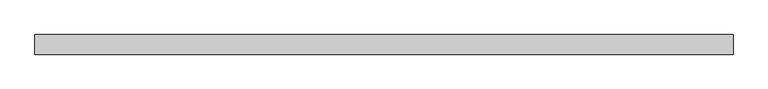
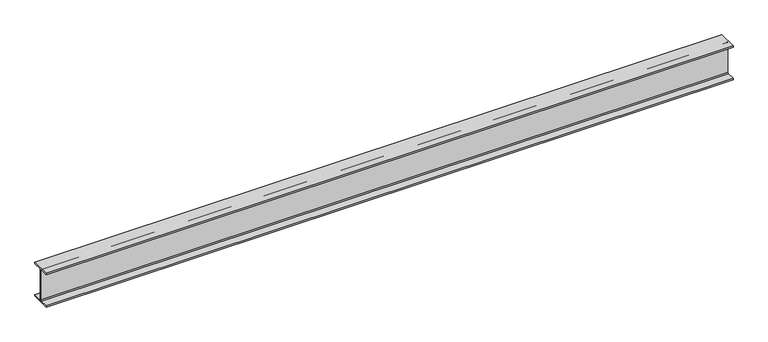
"""IFC4 building model written with IfcOpenShell, lengths in millimetres: beam geometry, Old_Steel Beam_H-KSD3502 : H_SB_ASB_H-482×300x11x15."""

from ifc_helpers import new_model, si_unit, point, frame, frame_2d, origin, place, context, project, spatial, polyline, circle_curve, trimmed, segment, composite_curve, outline, extrude, source, transform, mapped, element, save


def beam_c295454d(model_context):
    return source(origin(), model_context, "Body", "SweptSolid", [
        extrude(outline(composite_curve([segment(polyline([(82.5, -141.5), (82.5, -151.7), (-82.5, -151.7), (-82.5, -141.5), (-11.9, -141.5)]), True, "CONTINUOUS"), segment(trimmed(circle_curve(frame_2d((-11.9, -132.6)), 8.9), [point((-11.9, -141.5))], [point((-3.0, -132.6))], True, "CARTESIAN"), True, "CONTINUOUS"), segment(polyline([(-3.0, -132.6), (-3.0, 132.6)]), True, "CONTINUOUS"), segment(trimmed(circle_curve(frame_2d((-11.9, 132.6)), 8.9), [point((-3.0, 132.6))], [point((-11.9, 141.5))], True, "CARTESIAN"), True, "CONTINUOUS"), segment(polyline([(-11.9, 141.5), (-82.5, 141.5), (-82.5, 151.7), (82.5, 151.7), (82.5, 141.5), (11.9, 141.5)]), True, "CONTINUOUS"), segment(trimmed(circle_curve(frame_2d((11.9, 132.6)), 8.9), [point((11.9, 141.5))], [point((3.0, 132.6))], True, "CARTESIAN"), True, "CONTINUOUS"), segment(polyline([(3.0, 132.6), (3.0, -132.6)]), True, "CONTINUOUS"), segment(trimmed(circle_curve(frame_2d((11.9, -132.6)), 8.9), [point((3.0, -132.6))], [point((11.9, -141.5))], True, "CARTESIAN"), True, "CONTINUOUS"), segment(polyline([(11.9, -141.5), (82.5, -141.5)]), True, "CONTINUOUS")], self_intersect=False)), frame((-2939.3, 0.0, 0.0), z_axis=(1.0, 0.0, 0.0), x_axis=(0.0, 1.0, 0.0)), (0.0, 0.0, 1.0), 5878.6),
    ])


if __name__ == "__main__":
    model = new_model("IFC4")
    model_context = context("Model", 3, world=origin())
    ifc_project = project(units=[si_unit("LENGTHUNIT", "METRE", prefix="MILLI")], contexts=[model_context])
    site = spatial("IfcSite", under=ifc_project)
    building = spatial("IfcBuilding", under=site)
    placement = place(None, origin())
    beam_shape = beam_c295454d(model_context)
    element("IfcBeam", 1, ObjectType="Old_Steel Beam_H-KSD3502 : H_SB_ASB_H-482×300x11x15", at=placement, inside=building, context=model_context, shape_type="MappedRepresentation", body=[
        mapped(beam_shape, transform((0.0, 0.0, 0.0), x_axis=(1.0, 0.0, 0.0), y_axis=(0.0, 1.0, 0.0), z_axis=(0.0, 0.0, 1.0))),
    ])
    save(model, "model.ifc")

# Revit data of these elements
# Type "Old_Steel Beam_H-KSD3502 : H_SB_ASB_H-482×300x11x15"
#   Width = 30.0 cm
#   Web Thickness = 1.1 cm
#   Web Fillet = 2.6 cm
#   Warping Constant = 3680250.0 cm⁶
#   Torsional Moment of Inertia = 88.2192 cm⁴
#   Torsional Modulus = 1.0 cm³
#   Section Area = 145.5 cm²
#   Plastic Modulus weak axis = 695.0 cm³
#   Plastic Modulus strong axis = 2790.0 cm³
#   Perimeter = 2.10 m²/m
#   Nominal Weight = 114.00 kgf/m
#   Moment of Inertia weak axis = 6760.00 cm⁴
#   Moment of Inertia strong axis = 60400.00 cm⁴
#   Height = 48.2 cm
#   Flange Thickness = 1.5 cm
#   Elastic Modulus weak axis = 451.0 cm³
#   Elastic Modulus strong axis = 2500.0 cm³
#   Centroid Vertical = 24.1 cm
#   Centroid Horizontal = 15.0 cm
#   Length [instance default] = 1.5240 m
#   Structural Material [instance default] = Steel, 45-345
#   Assembly Code = ""
# Element 1 (IfcBeam, "Old_Steel Beam_H-KSD3502 : H_SB_ASB_H-482×300x11x15")
#   Structural Material = none
# Materials
#   "Steel, 45-345": class "Metal", colour RGB 189 187 185, transparency 0, Description = "Steel 345 MPa", Cost = 0
